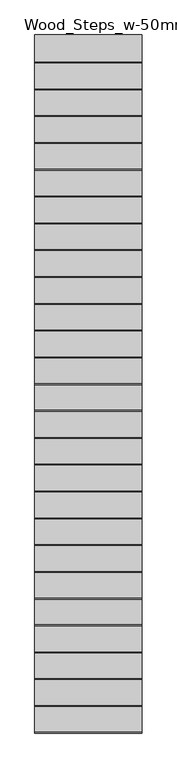
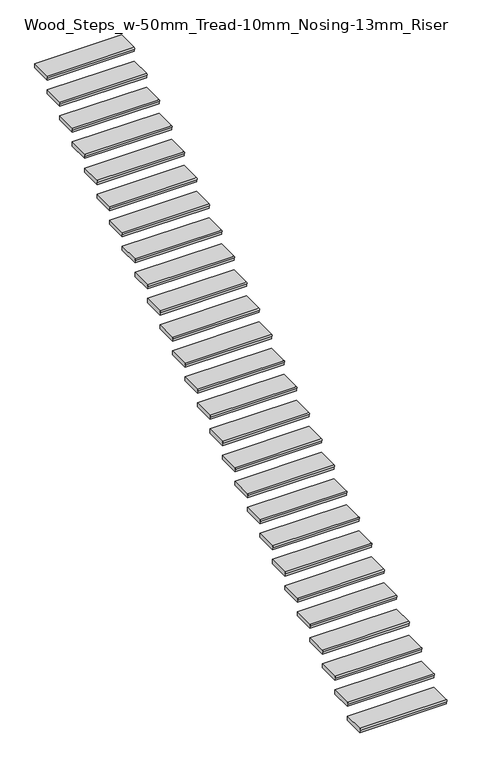
"""IFC4 building model written with IfcOpenShell, lengths in millimetres: stair flight geometry, Wood_Steps_w-50mm_Tread-10mm_Nosing-13mm_Riser."""

from ifc_helpers import new_model, si_unit, point, frame, frame_2d, origin, place, context, project, spatial, polyline, circle_curve, trimmed, segment, composite_curve, outline, extrude, source, transform, mapped, element, save


def wood_steps_w_50mm_tread_10mm_nosing_13mm_riser_36a02d2c(model_context):
    return source(origin(), model_context, "Body", "SweptSolid", [
        extrude(outline(composite_curve([segment(polyline([(-9742.8970515, 166.6666667), (-9492.8970515, 166.6666667), (-9492.8970515, 116.6666667), (-9742.8970515, 116.6666667), (-9742.8970515, 146.6666667)]), True, "CONTINUOUS"), segment(trimmed(circle_curve(frame_2d((-9742.8970515, 156.6666667)), 10.0), [point((-9742.8970515, 146.6666667))], [point((-9742.8970515, 166.6666667))], False, "CARTESIAN"), True, "CONTINUOUS")], self_intersect=False)), frame((-4553.6322783, 0.0, 0.0), z_axis=(1.0, 0.0, 0.0), x_axis=(0.0, 1.0, 0.0)), (0.0, 0.0, 1.0), 1000.0),
        extrude(outline(composite_curve([segment(polyline([(-9492.8970515, 333.3333333), (-9242.8970515, 333.3333333), (-9242.8970515, 283.3333333), (-9492.8970515, 283.3333333), (-9492.8970515, 313.3333333)]), True, "CONTINUOUS"), segment(trimmed(circle_curve(frame_2d((-9492.8970515, 323.3333333)), 10.0), [point((-9492.8970515, 313.3333333))], [point((-9492.8970515, 333.3333333))], False, "CARTESIAN"), True, "CONTINUOUS")], self_intersect=False)), frame((-4553.6322783, 0.0, 0.0), z_axis=(1.0, 0.0, 0.0), x_axis=(0.0, 1.0, 0.0)), (0.0, 0.0, 1.0), 1000.0),
        extrude(outline(composite_curve([segment(polyline([(-9242.8970515, 500.0), (-8992.8970515, 500.0), (-8992.8970515, 450.0), (-9242.8970515, 450.0), (-9242.8970515, 480.0)]), True, "CONTINUOUS"), segment(trimmed(circle_curve(frame_2d((-9242.8970515, 490.0)), 10.0), [point((-9242.8970515, 480.0))], [point((-9242.8970515, 500.0))], False, "CARTESIAN"), True, "CONTINUOUS")], self_intersect=False)), frame((-4553.6322783, 0.0, 0.0), z_axis=(1.0, 0.0, 0.0), x_axis=(0.0, 1.0, 0.0)), (0.0, 0.0, 1.0), 1000.0),
        extrude(outline(composite_curve([segment(polyline([(-8992.8970515, 666.6666667), (-8742.8970515, 666.6666667), (-8742.8970515, 616.6666667), (-8992.8970515, 616.6666667), (-8992.8970515, 646.6666667)]), True, "CONTINUOUS"), segment(trimmed(circle_curve(frame_2d((-8992.8970515, 656.6666667)), 10.0), [point((-8992.8970515, 646.6666667))], [point((-8992.8970515, 666.6666667))], False, "CARTESIAN"), True, "CONTINUOUS")], self_intersect=False)), frame((-4553.6322783, 0.0, 0.0), z_axis=(1.0, 0.0, 0.0), x_axis=(0.0, 1.0, 0.0)), (0.0, 0.0, 1.0), 1000.0),
        extrude(outline(composite_curve([segment(polyline([(-8742.8970515, 833.3333333), (-8492.8970515, 833.3333333), (-8492.8970515, 783.3333333), (-8742.8970515, 783.3333333), (-8742.8970515, 813.3333333)]), True, "CONTINUOUS"), segment(trimmed(circle_curve(frame_2d((-8742.8970515, 823.3333333)), 10.0), [point((-8742.8970515, 813.3333333))], [point((-8742.8970515, 833.3333333))], False, "CARTESIAN"), True, "CONTINUOUS")], self_intersect=False)), frame((-4553.6322783, 0.0, 0.0), z_axis=(1.0, 0.0, 0.0), x_axis=(0.0, 1.0, 0.0)), (0.0, 0.0, 1.0), 1000.0),
        extrude(outline(composite_curve([segment(polyline([(-8492.8970515, 1000.0), (-8242.8970515, 1000.0), (-8242.8970515, 950.0), (-8492.8970515, 950.0), (-8492.8970515, 980.0)]), True, "CONTINUOUS"), segment(trimmed(circle_curve(frame_2d((-8492.8970515, 990.0)), 10.0), [point((-8492.8970515, 980.0))], [point((-8492.8970515, 1000.0))], False, "CARTESIAN"), True, "CONTINUOUS")], self_intersect=False)), frame((-4553.6322783, 0.0, 0.0), z_axis=(1.0, 0.0, 0.0), x_axis=(0.0, 1.0, 0.0)), (0.0, 0.0, 1.0), 1000.0),
        extrude(outline(composite_curve([segment(polyline([(-8242.8970515, 1166.6666667), (-7992.8970515, 1166.6666667), (-7992.8970515, 1116.6666667), (-8242.8970515, 1116.6666667), (-8242.8970515, 1146.6666667)]), True, "CONTINUOUS"), segment(trimmed(circle_curve(frame_2d((-8242.8970515, 1156.6666667)), 10.0), [point((-8242.8970515, 1146.6666667))], [point((-8242.8970515, 1166.6666667))], False, "CARTESIAN"), True, "CONTINUOUS")], self_intersect=False)), frame((-4553.6322783, 0.0, 0.0), z_axis=(1.0, 0.0, 0.0), x_axis=(0.0, 1.0, 0.0)), (0.0, 0.0, 1.0), 1000.0),
        extrude(outline(composite_curve([segment(polyline([(-7992.8970515, 1333.3333333), (-7742.8970515, 1333.3333333), (-7742.8970515, 1283.3333333), (-7992.8970515, 1283.3333333), (-7992.8970515, 1313.3333333)]), True, "CONTINUOUS"), segment(trimmed(circle_curve(frame_2d((-7992.8970515, 1323.3333333)), 10.0), [point((-7992.8970515, 1313.3333333))], [point((-7992.8970515, 1333.3333333))], False, "CARTESIAN"), True, "CONTINUOUS")], self_intersect=False)), frame((-4553.6322783, 0.0, 0.0), z_axis=(1.0, 0.0, 0.0), x_axis=(0.0, 1.0, 0.0)), (0.0, 0.0, 1.0), 1000.0),
        extrude(outline(composite_curve([segment(polyline([(-7742.8970515, 1500.0), (-7492.8970515, 1500.0), (-7492.8970515, 1450.0), (-7742.8970515, 1450.0), (-7742.8970515, 1480.0)]), True, "CONTINUOUS"), segment(trimmed(circle_curve(frame_2d((-7742.8970515, 1490.0)), 10.0), [point((-7742.8970515, 1480.0))], [point((-7742.8970515, 1500.0))], False, "CARTESIAN"), True, "CONTINUOUS")], self_intersect=False)), frame((-4553.6322783, 0.0, 0.0), z_axis=(1.0, 0.0, 0.0), x_axis=(0.0, 1.0, 0.0)), (0.0, 0.0, 1.0), 1000.0),
        extrude(outline(composite_curve([segment(polyline([(-7492.8970515, 1666.6666667), (-7242.8970515, 1666.6666667), (-7242.8970515, 1616.6666667), (-7492.8970515, 1616.6666667), (-7492.8970515, 1646.6666667)]), True, "CONTINUOUS"), segment(trimmed(circle_curve(frame_2d((-7492.8970515, 1656.6666667)), 10.0), [point((-7492.8970515, 1646.6666667))], [point((-7492.8970515, 1666.6666667))], False, "CARTESIAN"), True, "CONTINUOUS")], self_intersect=False)), frame((-4553.6322783, 0.0, 0.0), z_axis=(1.0, 0.0, 0.0), x_axis=(0.0, 1.0, 0.0)), (0.0, 0.0, 1.0), 1000.0),
        extrude(outline(composite_curve([segment(polyline([(-7242.8970515, 1833.3333333), (-6992.8970515, 1833.3333333), (-6992.8970515, 1783.3333333), (-7242.8970515, 1783.3333333), (-7242.8970515, 1813.3333333)]), True, "CONTINUOUS"), segment(trimmed(circle_curve(frame_2d((-7242.8970515, 1823.3333333)), 10.0), [point((-7242.8970515, 1813.3333333))], [point((-7242.8970515, 1833.3333333))], False, "CARTESIAN"), True, "CONTINUOUS")], self_intersect=False)), frame((-4553.6322783, 0.0, 0.0), z_axis=(1.0, 0.0, 0.0), x_axis=(0.0, 1.0, 0.0)), (0.0, 0.0, 1.0), 1000.0),
        extrude(outline(composite_curve([segment(polyline([(-6992.8970515, 2000.0), (-6742.8970515, 2000.0), (-6742.8970515, 1950.0), (-6992.8970515, 1950.0), (-6992.8970515, 1980.0)]), True, "CONTINUOUS"), segment(trimmed(circle_curve(frame_2d((-6992.8970515, 1990.0)), 10.0), [point((-6992.8970515, 1980.0))], [point((-6992.8970515, 2000.0))], False, "CARTESIAN"), True, "CONTINUOUS")], self_intersect=False)), frame((-4553.6322783, 0.0, 0.0), z_axis=(1.0, 0.0, 0.0), x_axis=(0.0, 1.0, 0.0)), (0.0, 0.0, 1.0), 1000.0),
        extrude(outline(composite_curve([segment(polyline([(-6742.8970515, 2166.6666667), (-6492.8970515, 2166.6666667), (-6492.8970515, 2116.6666667), (-6742.8970515, 2116.6666667), (-6742.8970515, 2146.6666667)]), True, "CONTINUOUS"), segment(trimmed(circle_curve(frame_2d((-6742.8970515, 2156.6666667)), 10.0), [point((-6742.8970515, 2146.6666667))], [point((-6742.8970515, 2166.6666667))], False, "CARTESIAN"), True, "CONTINUOUS")], self_intersect=False)), frame((-4553.6322783, 0.0, 0.0), z_axis=(1.0, 0.0, 0.0), x_axis=(0.0, 1.0, 0.0)), (0.0, 0.0, 1.0), 1000.0),
        extrude(outline(composite_curve([segment(polyline([(-6492.8970515, 2333.3333333), (-6242.8970515, 2333.3333333), (-6242.8970515, 2283.3333333), (-6492.8970515, 2283.3333333), (-6492.8970515, 2313.3333333)]), True, "CONTINUOUS"), segment(trimmed(circle_curve(frame_2d((-6492.8970515, 2323.3333333)), 10.0), [point((-6492.8970515, 2313.3333333))], [point((-6492.8970515, 2333.3333333))], False, "CARTESIAN"), True, "CONTINUOUS")], self_intersect=False)), frame((-4553.6322783, 0.0, 0.0), z_axis=(1.0, 0.0, 0.0), x_axis=(0.0, 1.0, 0.0)), (0.0, 0.0, 1.0), 1000.0),
        extrude(outline(composite_curve([segment(polyline([(-6242.8970515, 2500.0), (-5992.8970515, 2500.0), (-5992.8970515, 2450.0), (-6242.8970515, 2450.0), (-6242.8970515, 2480.0)]), True, "CONTINUOUS"), segment(trimmed(circle_curve(frame_2d((-6242.8970515, 2490.0)), 10.0), [point((-6242.8970515, 2480.0))], [point((-6242.8970515, 2500.0))], False, "CARTESIAN"), True, "CONTINUOUS")], self_intersect=False)), frame((-4553.6322783, 0.0, 0.0), z_axis=(1.0, 0.0, 0.0), x_axis=(0.0, 1.0, 0.0)), (0.0, 0.0, 1.0), 1000.0),
        extrude(outline(composite_curve([segment(polyline([(-5992.8970515, 2666.6666667), (-5742.8970515, 2666.6666667), (-5742.8970515, 2616.6666667), (-5992.8970515, 2616.6666667), (-5992.8970515, 2646.6666667)]), True, "CONTINUOUS"), segment(trimmed(circle_curve(frame_2d((-5992.8970515, 2656.6666667)), 10.0), [point((-5992.8970515, 2646.6666667))], [point((-5992.8970515, 2666.6666667))], False, "CARTESIAN"), True, "CONTINUOUS")], self_intersect=False)), frame((-4553.6322783, 0.0, 0.0), z_axis=(1.0, 0.0, 0.0), x_axis=(0.0, 1.0, 0.0)), (0.0, 0.0, 1.0), 1000.0),
        extrude(outline(composite_curve([segment(polyline([(-5742.8970515, 2833.3333333), (-5492.8970515, 2833.3333333), (-5492.8970515, 2783.3333333), (-5742.8970515, 2783.3333333), (-5742.8970515, 2813.3333333)]), True, "CONTINUOUS"), segment(trimmed(circle_curve(frame_2d((-5742.8970515, 2823.3333333)), 10.0), [point((-5742.8970515, 2813.3333333))], [point((-5742.8970515, 2833.3333333))], False, "CARTESIAN"), True, "CONTINUOUS")], self_intersect=False)), frame((-4553.6322783, 0.0, 0.0), z_axis=(1.0, 0.0, 0.0), x_axis=(0.0, 1.0, 0.0)), (0.0, 0.0, 1.0), 1000.0),
        extrude(outline(composite_curve([segment(polyline([(-5492.8970515, 3000.0), (-5242.8970515, 3000.0), (-5242.8970515, 2950.0), (-5492.8970515, 2950.0), (-5492.8970515, 2980.0)]), True, "CONTINUOUS"), segment(trimmed(circle_curve(frame_2d((-5492.8970515, 2990.0)), 10.0), [point((-5492.8970515, 2980.0))], [point((-5492.8970515, 3000.0))], False, "CARTESIAN"), True, "CONTINUOUS")], self_intersect=False)), frame((-4553.6322783, 0.0, 0.0), z_axis=(1.0, 0.0, 0.0), x_axis=(0.0, 1.0, 0.0)), (0.0, 0.0, 1.0), 1000.0),
        extrude(outline(composite_curve([segment(polyline([(-5242.8970515, 3166.6666667), (-4992.8970515, 3166.6666667), (-4992.8970515, 3116.6666667), (-5242.8970515, 3116.6666667), (-5242.8970515, 3146.6666667)]), True, "CONTINUOUS"), segment(trimmed(circle_curve(frame_2d((-5242.8970515, 3156.6666667)), 10.0), [point((-5242.8970515, 3146.6666667))], [point((-5242.8970515, 3166.6666667))], False, "CARTESIAN"), True, "CONTINUOUS")], self_intersect=False)), frame((-4553.6322783, 0.0, 0.0), z_axis=(1.0, 0.0, 0.0), x_axis=(0.0, 1.0, 0.0)), (0.0, 0.0, 1.0), 1000.0),
        extrude(outline(composite_curve([segment(polyline([(-4992.8970515, 3333.3333333), (-4742.8970515, 3333.3333333), (-4742.8970515, 3283.3333333), (-4992.8970515, 3283.3333333), (-4992.8970515, 3313.3333333)]), True, "CONTINUOUS"), segment(trimmed(circle_curve(frame_2d((-4992.8970515, 3323.3333333)), 10.0), [point((-4992.8970515, 3313.3333333))], [point((-4992.8970515, 3333.3333333))], False, "CARTESIAN"), True, "CONTINUOUS")], self_intersect=False)), frame((-4553.6322783, 0.0, 0.0), z_axis=(1.0, 0.0, 0.0), x_axis=(0.0, 1.0, 0.0)), (0.0, 0.0, 1.0), 1000.0),
        extrude(outline(composite_curve([segment(polyline([(-4742.8970515, 3500.0), (-4492.8970515, 3500.0), (-4492.8970515, 3450.0), (-4742.8970515, 3450.0), (-4742.8970515, 3480.0)]), True, "CONTINUOUS"), segment(trimmed(circle_curve(frame_2d((-4742.8970515, 3490.0)), 10.0), [point((-4742.8970515, 3480.0))], [point((-4742.8970515, 3500.0))], False, "CARTESIAN"), True, "CONTINUOUS")], self_intersect=False)), frame((-4553.6322783, 0.0, 0.0), z_axis=(1.0, 0.0, 0.0), x_axis=(0.0, 1.0, 0.0)), (0.0, 0.0, 1.0), 1000.0),
        extrude(outline(composite_curve([segment(polyline([(-4492.8970515, 3666.6666667), (-4242.8970515, 3666.6666667), (-4242.8970515, 3616.6666667), (-4492.8970515, 3616.6666667), (-4492.8970515, 3646.6666667)]), True, "CONTINUOUS"), segment(trimmed(circle_curve(frame_2d((-4492.8970515, 3656.6666667)), 10.0), [point((-4492.8970515, 3646.6666667))], [point((-4492.8970515, 3666.6666667))], False, "CARTESIAN"), True, "CONTINUOUS")], self_intersect=False)), frame((-4553.6322783, 0.0, 0.0), z_axis=(1.0, 0.0, 0.0), x_axis=(0.0, 1.0, 0.0)), (0.0, 0.0, 1.0), 1000.0),
        extrude(outline(composite_curve([segment(polyline([(-4242.8970515, 3833.3333333), (-3992.8970515, 3833.3333333), (-3992.8970515, 3783.3333333), (-4242.8970515, 3783.3333333), (-4242.8970515, 3813.3333333)]), True, "CONTINUOUS"), segment(trimmed(circle_curve(frame_2d((-4242.8970515, 3823.3333333)), 10.0), [point((-4242.8970515, 3813.3333333))], [point((-4242.8970515, 3833.3333333))], False, "CARTESIAN"), True, "CONTINUOUS")], self_intersect=False)), frame((-4553.6322783, 0.0, 0.0), z_axis=(1.0, 0.0, 0.0), x_axis=(0.0, 1.0, 0.0)), (0.0, 0.0, 1.0), 1000.0),
        extrude(outline(composite_curve([segment(polyline([(-3992.8970515, 4000.0), (-3742.8970515, 4000.0), (-3742.8970515, 3950.0), (-3992.8970515, 3950.0), (-3992.8970515, 3980.0)]), True, "CONTINUOUS"), segment(trimmed(circle_curve(frame_2d((-3992.8970515, 3990.0)), 10.0), [point((-3992.8970515, 3980.0))], [point((-3992.8970515, 4000.0))], False, "CARTESIAN"), True, "CONTINUOUS")], self_intersect=False)), frame((-4553.6322783, 0.0, 0.0), z_axis=(1.0, 0.0, 0.0), x_axis=(0.0, 1.0, 0.0)), (0.0, 0.0, 1.0), 1000.0),
        extrude(outline(composite_curve([segment(polyline([(-3742.8970515, 4166.6666667), (-3492.8970515, 4166.6666667), (-3492.8970515, 4116.6666667), (-3742.8970515, 4116.6666667), (-3742.8970515, 4146.6666667)]), True, "CONTINUOUS"), segment(trimmed(circle_curve(frame_2d((-3742.8970515, 4156.6666667)), 10.0), [point((-3742.8970515, 4146.6666667))], [point((-3742.8970515, 4166.6666667))], False, "CARTESIAN"), True, "CONTINUOUS")], self_intersect=False)), frame((-4553.6322783, 0.0, 0.0), z_axis=(1.0, 0.0, 0.0), x_axis=(0.0, 1.0, 0.0)), (0.0, 0.0, 1.0), 1000.0),
        extrude(outline(composite_curve([segment(polyline([(-3492.8970515, 4333.3333333), (-3242.8970515, 4333.3333333), (-3242.8970515, 4283.3333333), (-3492.8970515, 4283.3333333), (-3492.8970515, 4313.3333333)]), True, "CONTINUOUS"), segment(trimmed(circle_curve(frame_2d((-3492.8970515, 4323.3333333)), 10.0), [point((-3492.8970515, 4313.3333333))], [point((-3492.8970515, 4333.3333333))], False, "CARTESIAN"), True, "CONTINUOUS")], self_intersect=False)), frame((-4553.6322783, 0.0, 0.0), z_axis=(1.0, 0.0, 0.0), x_axis=(0.0, 1.0, 0.0)), (0.0, 0.0, 1.0), 1000.0),
    ])


if __name__ == "__main__":
    model = new_model("IFC4")
    model_context = context("Model", 3, world=origin())
    ifc_project = project(units=[si_unit("LENGTHUNIT", "METRE", prefix="MILLI")], contexts=[model_context])
    site = spatial("IfcSite", under=ifc_project)
    building = spatial("IfcBuilding", under=site)
    placement = place(None, origin())
    wood_steps_w_50mm_tread_10mm_nosing_13mm_riser_shape = wood_steps_w_50mm_tread_10mm_nosing_13mm_riser_36a02d2c(model_context)
    element("IfcStairFlight", 1, ObjectType="Wood_Steps_w-50mm_Tread-10mm_Nosing-13mm_Riser", at=placement, inside=building, context=model_context, shape_type="MappedRepresentation", body=[
        mapped(wood_steps_w_50mm_tread_10mm_nosing_13mm_riser_shape, transform((0.0, 0.0, 0.0), x_axis=(1.0, 0.0, 0.0), y_axis=(0.0, 1.0, 0.0), z_axis=(0.0, 0.0, 1.0))),
    ])
    save(model, "model.ifc")

# Revit data of these elements
# Element 1 (IfcStairFlight, "Wood_Steps_w-50mm_Tread-10mm_Nosing-13mm_Riser")
#   Materials on its faces: "Oak Flooring"
# Materials
#   "Oak Flooring": class "Wood", colour RGB 212 179 113, transparency 0, Description = "Quercus Rubra", Cost = 0
